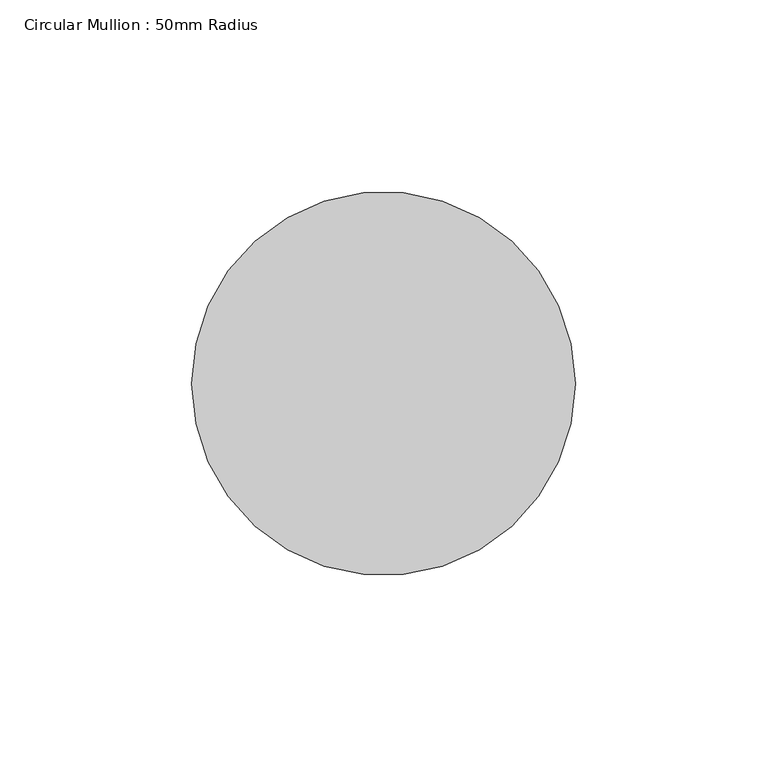
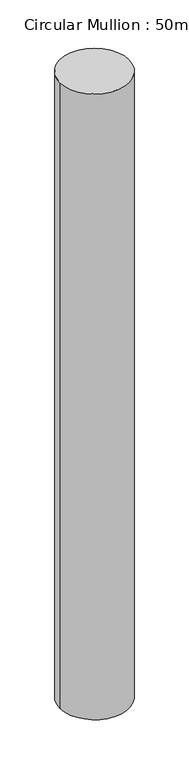
"""IFC4 building model written with IfcOpenShell, lengths in millimetres: member geometry, Circular Mullion : 50mm Radius."""

from ifc_helpers import new_model, si_unit, point, frame, origin, origin_2d, place, context, project, spatial, circle_curve, trimmed, segment, composite_curve, outline, extrude, source, transform, mapped, element, save


def circular_mullion_50mm_radius_0d07fdbf(model_context):
    return source(origin(), model_context, "Body", "SweptSolid", [
        extrude(outline(composite_curve([segment(trimmed(circle_curve(origin_2d(), 50.0), [point((50.0, 0.0))], [point((-50.0, 0.0))], False, "CARTESIAN"), True, "CONTINUOUS"), segment(trimmed(circle_curve(origin_2d(), 50.0), [point((-50.0, 0.0))], [point((50.0, 0.0))], False, "CARTESIAN"), True, "CONTINUOUS")], self_intersect=False)), frame((0.0, 0.0, -957.5156209), z_axis=(0.0, 0.0, 1.0), x_axis=(1.0, 0.0, 0.0)), (0.0, 0.0, 1.0), 957.5156209),
    ])


if __name__ == "__main__":
    model = new_model("IFC4")
    model_context = context("Model", 3, world=origin())
    ifc_project = project(units=[si_unit("LENGTHUNIT", "METRE", prefix="MILLI")], contexts=[model_context])
    site = spatial("IfcSite", under=ifc_project)
    building = spatial("IfcBuilding", under=site)
    placement = place(None, origin())
    circular_mullion_50mm_radius_shape = circular_mullion_50mm_radius_0d07fdbf(model_context)
    element("IfcMember", 1, ObjectType="Circular Mullion : 50mm Radius", at=placement, inside=building, context=model_context, shape_type="MappedRepresentation", body=[
        mapped(circular_mullion_50mm_radius_shape, transform((0.0, 0.0, 0.0), x_axis=(1.0, 0.0, 0.0), y_axis=(0.0, 1.0, 0.0), z_axis=(0.0, 0.0, 1.0))),
    ])
    save(model, "model.ifc")

# Revit data of these elements
# Type "Circular Mullion : 50mm Radius"
#   built-in parameter 1007350 = 0.164042 (stored number, unit not read)
# Element 1 (IfcMember, "Circular Mullion : 50mm Radius")
#   Materials on its faces: "Aluminium"
# Materials
#   "Aluminium": class "Metal", colour RGB 247 247 247, transparency 0, Description = "Aluminium 6061", Cost = 0
